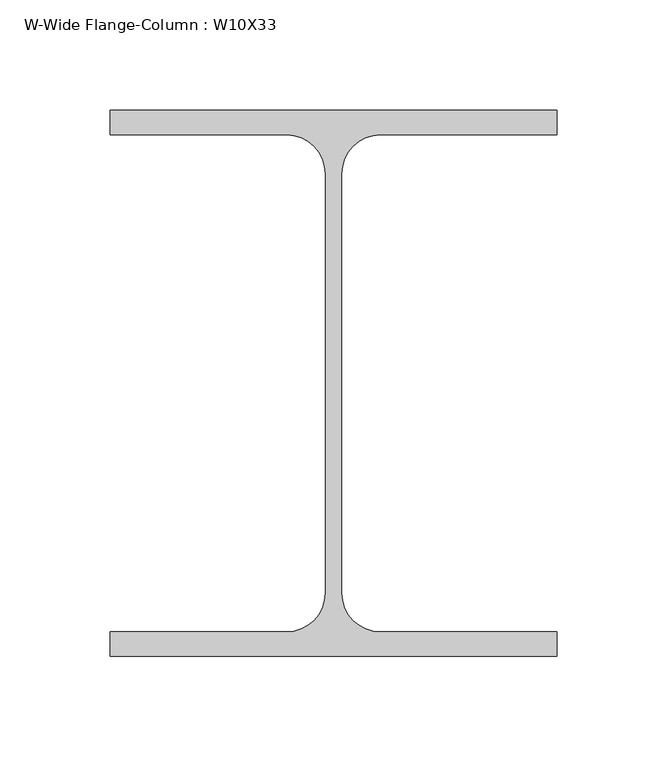
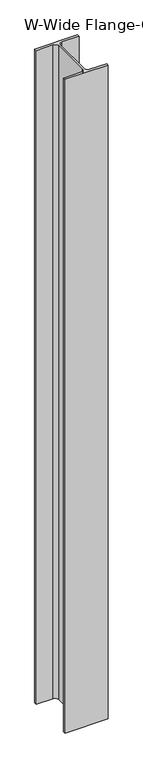
"""IFC4 building model written with IfcOpenShell, lengths in millimetres: column geometry, W-Wide Flange-Column : W10X33."""

from ifc_helpers import new_model, si_unit, point, frame, frame_2d, origin, place, context, project, spatial, polyline, circle_curve, trimmed, segment, composite_curve, outline, extrude, source, transform, mapped, element, save


def w_wide_flange_column_w10x33_c392bb88(model_context):
    return source(origin(), model_context, "Body", "SweptSolid", [
        extrude(outline(composite_curve([segment(polyline([(101.092, 123.571), (101.092, 112.522), (21.209, 112.522)]), True, "CONTINUOUS"), segment(trimmed(circle_curve(frame_2d((21.209, 94.996)), 17.526), [point((21.209, 112.522))], [point((3.683, 94.996))], True, "CARTESIAN"), True, "CONTINUOUS"), segment(polyline([(3.683, 94.996), (3.683, -94.996)]), True, "CONTINUOUS"), segment(trimmed(circle_curve(frame_2d((21.209, -94.996)), 17.526), [point((3.683, -94.996))], [point((21.209, -112.522))], True, "CARTESIAN"), True, "CONTINUOUS"), segment(polyline([(21.209, -112.522), (101.092, -112.522), (101.092, -123.571), (-101.092, -123.571), (-101.092, -112.522), (-21.209, -112.522)]), True, "CONTINUOUS"), segment(trimmed(circle_curve(frame_2d((-21.209, -94.996)), 17.526), [point((-21.209, -112.522))], [point((-3.683, -94.996))], True, "CARTESIAN"), True, "CONTINUOUS"), segment(polyline([(-3.683, -94.996), (-3.683, 94.996)]), True, "CONTINUOUS"), segment(trimmed(circle_curve(frame_2d((-21.209, 94.996)), 17.526), [point((-3.683, 94.996))], [point((-21.209, 112.522))], True, "CARTESIAN"), True, "CONTINUOUS"), segment(polyline([(-21.209, 112.522), (-101.092, 112.522), (-101.092, 123.571), (101.092, 123.571)]), True, "CONTINUOUS")], self_intersect=False)), frame((0.0, 0.0, 9163.05), z_axis=(0.0, 0.0, 1.0), x_axis=(1.0, 0.0, 0.0)), (0.0, 0.0, 1.0), 3244.85),
    ])


if __name__ == "__main__":
    model = new_model("IFC4")
    model_context = context("Model", 3, world=origin())
    ifc_project = project(units=[si_unit("LENGTHUNIT", "METRE", prefix="MILLI")], contexts=[model_context])
    site = spatial("IfcSite", under=ifc_project)
    building = spatial("IfcBuilding", under=site)
    placement = place(None, origin())
    w_wide_flange_column_w10x33_shape = w_wide_flange_column_w10x33_c392bb88(model_context)
    element("IfcColumn", 1, ObjectType="W-Wide Flange-Column : W10X33", at=placement, inside=building, context=model_context, shape_type="MappedRepresentation", body=[
        mapped(w_wide_flange_column_w10x33_shape, transform((0.0, 0.0, 0.0), x_axis=(1.0, 0.0, 0.0), y_axis=(0.0, 1.0, 0.0), z_axis=(0.0, 0.0, 1.0))),
    ])
    save(model, "model.ifc")

# Revit data of these elements
# Type "W-Wide Flange-Column : W10X33"
#   Assembly Code = "B10"
#   W = 33
#   bf = 0' - 7.96"
#   d = 0' - 9.73"
#   k = 0' - 1 1/8"
#   kr = 0' - 0.69"
#   tf = 0' - 0.435"
#   tw = 0' - 0.29"
#   A = 0.0674306 SF
#   Structural Material [instance default] = Steel ASTM A992
# Element 1 (IfcColumn, "W-Wide Flange-Column : W10X33")
#   Materials on its faces: "Steel ASTM A992"
# Materials
#   "Steel ASTM A992": class "Metal", colour RGB 199 199 199, transparency 0, Description = "Structural steel 50ksi", Cost = 0
